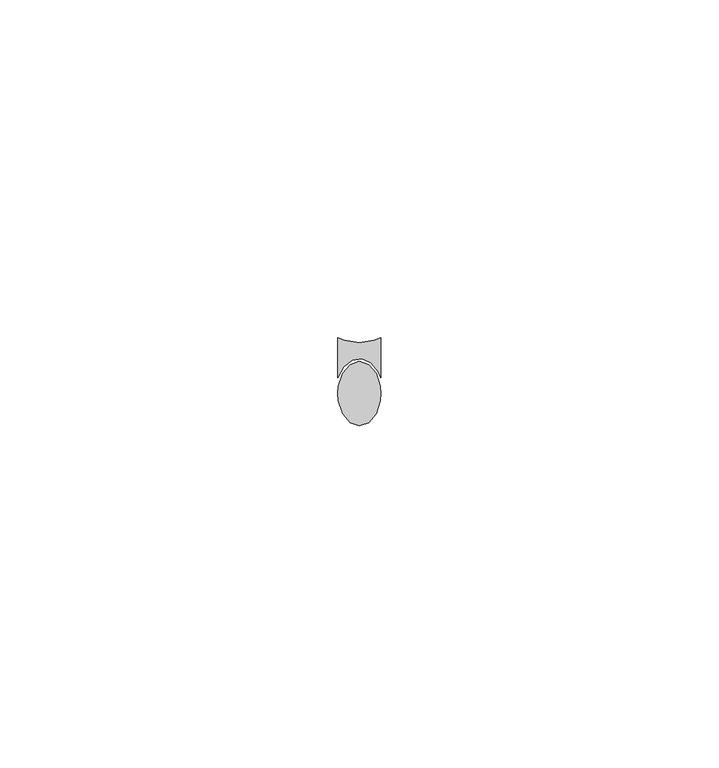
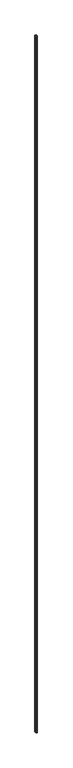
"""IFC4 building model written with IfcOpenShell, lengths in millimetres: proxy geometry, Generic Models 11:Generic Models 1:306267:Generic Models 1:306267 : Generic Models 11:Generic Models 1:306267:300405:Generic Models 1:306267:Generic Models 1:306267 : Generic Models 11:Generic Models 1:306267:300405 : Generic Models 11:Generic Models 1:306267:Generic Models 1:306267 : Generic Models 11:Generic Models 1:306267:300405:16 : Generic Models 11:Generic Models 1:306267:Generic Models 1:306267 : Generic Models 11:Generic Models 1:306267:300405:Generic Models 1:306267:Generic Models 1:306267 : Generic Models 11:Generic Models 1:306267:300405 : Generic Models 11:Generic Models 1:306267:Generic Models 1:306267 : Generic Models 11:Generic Models 1:306267:300405:300182."""

from ifc_helpers import new_model, si_unit, origin, origin_with_axes, place, context, project, spatial, polyline, outline, extrude, source, transform, mapped, element, save


def generic_models_b16b8935(model_context):
    return source(origin(), model_context, "Body", "SweptSolid", [
        extrude(outline(polyline([(582706.3393048, -579036.3403513), (582707.4440389, -579037.6618453), (582708.0571201, -579039.5714595), (582708.1367239, -579040.6312155), (582708.0571201, -579041.6909714), (582707.4440389, -579043.6005857), (582706.3393048, -579044.9220797), (582704.9617239, -579045.3937155), (582703.5841431, -579044.9220797), (582702.479409, -579043.6005857), (582701.8663278, -579041.6909714), (582701.7867239, -579040.6312155), (582701.8663278, -579039.5714595), (582702.479409, -579037.6618453), (582703.5841431, -579036.3403513), (582704.9617239, -579035.8687155), (582706.3393048, -579036.3403513)])), origin_with_axes(), (0.0, 0.0, 1.0), 3695.7),
        extrude(outline(polyline([(582702.7524872, -579032.7769044), (582704.9617239, -579033.0905905), (582707.1709607, -579032.7769044), (582708.1367239, -579032.3994958), (582708.1367239, -579038.2675879), (582707.7504064, -579037.4073069), (582706.6669209, -579036.0977318), (582705.3166731, -579035.4973783), (582703.9108969, -579035.7001662), (582702.6695128, -579036.6743712), (582701.7867239, -579038.2675879), (582701.7867239, -579032.3994958), (582702.7524872, -579032.7769044)])), origin_with_axes(), (0.0, 0.0, 1.0), 3695.7),
    ])


if __name__ == "__main__":
    model = new_model("IFC4")
    model_context = context("Model", 3, world=origin())
    ifc_project = project(units=[si_unit("LENGTHUNIT", "METRE", prefix="MILLI")], contexts=[model_context])
    site = spatial("IfcSite", under=ifc_project)
    building = spatial("IfcBuilding", under=site)
    placement = place(None, origin())
    generic_models_shape = generic_models_b16b8935(model_context)
    element("IfcBuildingElementProxy", 1, Name="Generic Models 11:Generic Models 1:306267:Generic Models 1:306267 : Generic Models 11:Generic Models 1:306267:300405:Generic Models 1:306267:Generic Models 1:306267 : Generic Models 11:Generic Models 1:306267:300405 : Generic Models 11:Generic Models 1:306267:Generic Models 1:306267 : Generic Models 11:Generic Models 1:306267:300405:16 : Generic Models 11:Generic Models 1:306267:Generic Models 1:306267 : Generic Models 11:Generic Models 1:306267:300405:Generic Models 1:306267:Generic Models 1:306267 : Generic Models 11:Generic Models 1:306267:300405 : Generic Models 11:Generic Models 1:306267:Generic Models 1:306267 : Generic Models 11:Generic Models 1:306267:300405:300182", ObjectType="Generic Models 11:Generic Models 1:306267:Generic Models 1:306267 : Generic Models 11:Generic Models 1:306267:300405:Generic Models 1:306267:Generic Models 1:306267 : Generic Models 11:Generic Models 1:306267:300405 : Generic Models 11:Generic Models 1:306267:Generic Models 1:306267 : Generic Models 11:Generic Models 1:306267:300405:16 : Generic Models 11:Generic Models 1:306267:Generic Models 1:306267 : Generic Models 11:Generic Models 1:306267:300405:Generic Models 1:306267:Generic Models 1:306267 : Generic Models 11:Generic Models 1:306267:300405 : Generic Models 11:Generic Models 1:306267:Generic Models 1:306267 : Generic Models 11:Generic Models 1:306267:300405:300182", at=placement, inside=building, context=model_context, shape_type="MappedRepresentation", body=[
        mapped(generic_models_shape, transform((0.0, 0.0, 0.0), x_axis=(1.0, 0.0, 0.0), y_axis=(0.0, 1.0, 0.0), z_axis=(0.0, 0.0, 1.0))),
    ])
    save(model, "model.ifc")

# Revit data of these elements
# Type "Generic Models 11:Generic Models 1:306267:Generic Models 1:306267 : Generic Models 11:Generic Models 1:306267:300405:Generic Models 1:306267:Generic Models 1:306267 : Generic Models 11:Generic Models 1:306267:300405 : Generic Models 11:Generic Models 1:306267:Generic Models 1:306267 : Generic Models 11:Generic Models 1:306267:300405:16 : Generic Models 11:Generic Models 1:306267:Generic Models 1:306267 : Generic Models 11:Generic Models 1:306267:300405:Generic Models 1:306267:Generic Models 1:306267 : Generic Models 11:Generic Models 1:306267:300405 : Generic Models 11:Generic Models 1:306267:Generic Models 1:306267 : Generic Models 11:Generic Models 1:306267:300405:300182"
#   NameOverride = "Generic Models 11:Generic Models 1:306267:Generic Models 1:306267 : Generic Models 11:Generic Models 1:306267:300405:Generic Models 1:306267:Generic Models 1:306267 : Generic Models 11:Generic Models 1:306267:300405 : Generic Models 11:Generic Models 1:306267:Generic Models 1:306267 : Generic Models 11:Generic Models 1:306267:300405:300182"
#   ObjectTypeOverride = "Generic Models 1:306267:Generic Models 1:306267 : Generic Models 11:Generic Models 1:306267:300405 : Generic Models 11:Generic Models 1:306267:Generic Models 1:306267 : Generic Models 11:Generic Models 1:306267:300405"
#   Reference = "Generic Models 1"
#   Tag = "300182"
# Element 1 (IfcBuildingElementProxy, "Generic Models 11:Generic Models 1:306267:Generic Models 1:306267 : Generic Models 11:Generic Models 1:306267:300405:Generic Models 1:306267:Generic Models 1:306267 : Generic Models 11:Generic Models 1:306267:300405 : Generic Models 11:Generic Models 1:306267:Generic Models 1:306267 : Generic Models 11:Generic Models 1:306267:300405:16 : Generic Models 11:Generic Models 1:306267:Generic Models 1:306267 : Generic Models 11:Generic Models 1:306267:300405:Generic Models 1:306267:Generic Models 1:306267 : Generic Models 11:Generic Models 1:306267:300405 : Generic Models 11:Generic Models 1:306267:Generic Models 1:306267 : Generic Models 11:Generic Models 1:306267:300405:300182")
#   Materials on its faces: "SEALANT & BACKER ROD"
# Materials
#   "SEALANT & BACKER ROD": class "Unassigned", colour RGB 120 120 120, transparency 0, Cost = 0
